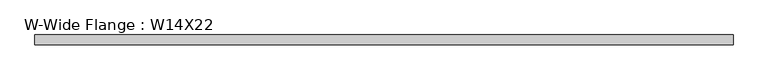
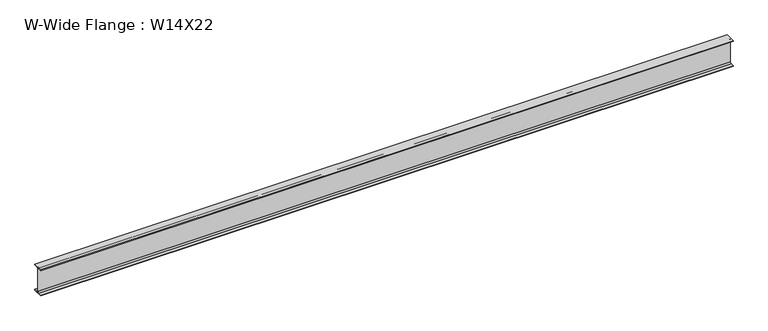
"""IFC4 building model written with IfcOpenShell, lengths in millimetres: beam geometry, W-Wide Flange : W14X22."""

import ifcopenshell
import ifcopenshell.guid

model = None  # the IFC model being written
_history = None  # IfcOwnerHistory: only IFC2X3 demands one
_inside = {}  # id of a spatial element -> (the spatial element, [elements in it])
_under = {}  # id of a project, library or spatial element -> (it, [spatial elements below it])
_declared = {}  # id of a project -> (the project, [libraries it declares])
_typed = {}  # id of a type object -> (the type object, [elements of that type])
_made_of = {}  # id of a material, layer set ... -> (it, [elements and type objects made of it])


def new_model(schema):
    """Start an empty IFC model of exactly this schema.

    Asked for "IFC4X3", IfcOpenShell would pick the latest addendum, in which some entities
    have other attributes; the version numbers below select the first issue.
    IFC2X3 requires an IfcOwnerHistory on every rooted entity: one is made here for all.
    """
    global model, _history
    if schema == "IFC4X3":
        model = ifcopenshell.file(schema_version=(4, 3, 0, 0))
    else:
        model = ifcopenshell.file(schema=schema)
    _inside.clear()
    _under.clear()
    _declared.clear()
    _typed.clear()
    _made_of.clear()
    _history = None
    if model.schema == "IFC2X3":
        org = make("IfcOrganization", Name="unknown")
        user = make(
            "IfcPersonAndOrganization",
            ThePerson=make("IfcPerson", FamilyName="unknown"),
            TheOrganization=org,
        )
        app = make(
            "IfcApplication",
            ApplicationDeveloper=org,
            Version="unknown",
            ApplicationFullName="unknown",
            ApplicationIdentifier="unknown",
        )
        _history = make(
            "IfcOwnerHistory",
            OwningUser=user,
            OwningApplication=app,
            ChangeAction="ADDED",
            CreationDate=0,
        )
    return model


def make(cls, **values):
    """One entity of the class cls with the attributes given. An attribute that is None is left unset."""
    return model.create_entity(
        cls, **{name: value for name, value in values.items() if value is not None}
    )


def rooted(cls, **values):
    """An entity with a GlobalId (a new one), such as an element, a storey or a relation."""
    return make(cls, GlobalId=ifcopenshell.guid.new(), OwnerHistory=_history, **values)


def si_unit(unit_type, name, prefix=None):
    """IfcSIUnit, for example si_unit("LENGTHUNIT", "METRE", prefix="MILLI")."""
    return make("IfcSIUnit", UnitType=unit_type, Prefix=prefix, Name=name)


def assignment(units):
    """IfcUnitAssignment: the units of a project."""
    return None if units is None else make("IfcUnitAssignment", Units=units)


def point(xyz):
    """IfcCartesianPoint."""
    return None if xyz is None else make("IfcCartesianPoint", Coordinates=xyz)


def direction(xyz):
    """IfcDirection."""
    return None if xyz is None else make("IfcDirection", DirectionRatios=xyz)


def frame(location, z_axis=None, x_axis=None):
    """IfcAxis2Placement3D, a coordinate frame: its origin and axes. An axis left out is left unset."""
    return make(
        "IfcAxis2Placement3D",
        Location=point(location),
        Axis=direction(z_axis),
        RefDirection=direction(x_axis),
    )


def frame_2d(location, x_axis=None):
    """IfcAxis2Placement2D, a coordinate frame in the plane: its origin and x axis."""
    return make(
        "IfcAxis2Placement2D", Location=point(location), RefDirection=direction(x_axis)
    )


def origin():
    """The frame at (0, 0, 0) with its axes left unset."""
    return frame((0.0, 0.0, 0.0))


def place(relative_to, where):
    """IfcLocalPlacement: puts the frame where relative to a parent placement (None: the world)."""
    return make(
        "IfcLocalPlacement", PlacementRelTo=relative_to, RelativePlacement=where
    )


def context(
    kind, dimensions, precision=None, world=None, true_north=None, identifier=None
):
    """IfcGeometricRepresentationContext, for example the 3D "Model" context."""
    return make(
        "IfcGeometricRepresentationContext",
        ContextIdentifier=identifier,
        ContextType=kind,
        CoordinateSpaceDimension=dimensions,
        Precision=precision,
        WorldCoordinateSystem=world,
        TrueNorth=true_north,
    )


def project(units=None, contexts=None):
    """IfcProject with its units and contexts."""
    return rooted(
        "IfcProject",
        Name="project",
        RepresentationContexts=contexts,
        UnitsInContext=assignment(units),
    )


def spatial(cls, under=None, at=None, **own):
    """A site, building, storey or space (cls), placed at a placement, below another one or the project."""
    s = rooted(cls, ObjectPlacement=at, **own)
    if under is not None:
        _under.setdefault(under.id(), (under, []))[1].append(s)
    return s


def polyline(points):
    """IfcPolyline through the points."""
    return make("IfcPolyline", Points=[point(p) for p in points])


def circle_curve(where, radius):
    """IfcCircle in the frame where."""
    return make("IfcCircle", Position=where, Radius=radius)


def trimmed(basis, trim1, trim2, sense, master):
    """IfcTrimmedCurve: the piece of a basis curve between two trims."""
    return make(
        "IfcTrimmedCurve",
        BasisCurve=basis,
        Trim1=trim1,
        Trim2=trim2,
        SenseAgreement=sense,
        MasterRepresentation=master,
    )


def segment(curve, same_sense, transition):
    """IfcCompositeCurveSegment."""
    return make(
        "IfcCompositeCurveSegment",
        Transition=transition,
        SameSense=same_sense,
        ParentCurve=curve,
    )


def composite_curve(segments, self_intersect=None):
    """IfcCompositeCurve: segments joined end to end."""
    return make("IfcCompositeCurve", Segments=segments, SelfIntersect=self_intersect)


def outline(outer, holes=None, kind="AREA"):
    """IfcArbitraryClosedProfileDef: a profile drawn as a closed curve; with holes, ...WithVoids."""
    if holes is None:
        return make("IfcArbitraryClosedProfileDef", ProfileType=kind, OuterCurve=outer)
    return make(
        "IfcArbitraryProfileDefWithVoids",
        ProfileType=kind,
        OuterCurve=outer,
        InnerCurves=holes,
    )


def extrude(swept, where, along, depth):
    """IfcExtrudedAreaSolid: the profile swept, set in the frame where, extruded along a direction by depth."""
    return make(
        "IfcExtrudedAreaSolid",
        SweptArea=swept,
        Position=where,
        ExtrudedDirection=direction(along),
        Depth=depth,
    )


def shape(context_of_items, identifier, shape_type, items):
    """IfcShapeRepresentation: the items that make up one representation, for example the "Body"."""
    return make(
        "IfcShapeRepresentation",
        ContextOfItems=context_of_items,
        RepresentationIdentifier=identifier,
        RepresentationType=shape_type,
        Items=items,
    )


def source(mapping_origin, context_of_items, identifier, shape_type, items):
    """IfcRepresentationMap: a shape defined once, which mapped items show again and again."""
    return make(
        "IfcRepresentationMap",
        MappingOrigin=mapping_origin,
        MappedRepresentation=shape(context_of_items, identifier, shape_type, items),
    )


def transform(
    local_origin,
    x_axis=None,
    y_axis=None,
    z_axis=None,
    scale=None,
    scale2=None,
    scale3=None,
    uniform=True,
):
    """IfcCartesianTransformationOperator3D, or its non-uniform kind. x_axis, y_axis, z_axis: its Axis1, 2, 3."""
    if uniform:
        return make(
            "IfcCartesianTransformationOperator3D",
            Axis1=direction(x_axis),
            Axis2=direction(y_axis),
            LocalOrigin=point(local_origin),
            Scale=scale,
            Axis3=direction(z_axis),
        )
    return make(
        "IfcCartesianTransformationOperator3DnonUniform",
        Axis1=direction(x_axis),
        Axis2=direction(y_axis),
        LocalOrigin=point(local_origin),
        Scale=scale,
        Axis3=direction(z_axis),
        Scale2=scale2,
        Scale3=scale3,
    )


def mapped(mapping_source, mapping_target):
    """IfcMappedItem: shows the shape of a source again, moved by a transform."""
    return make(
        "IfcMappedItem", MappingSource=mapping_source, MappingTarget=mapping_target
    )


def made_of(thing, what):
    """Note that an element or type object is made of a material, layer set ...; save() writes the relation."""
    if what is not None:
        _made_of.setdefault(what.id(), (what, []))[1].append(thing)
    return thing


def element(
    cls,
    number,
    at=None,
    inside=None,
    cuts=None,
    type_object=None,
    material=None,
    context=None,
    identifier="Body",
    shape_type=None,
    held_by="IfcProductDefinitionShape",
    body=None,
    shapes=None,
    **own,
):
    """One element of the class cls, such as IfcWall. Its Tag is "e" and its number.

    at: its placement. inside: the storey or other place that contains it. cuts: it is an
    opening in that element (IfcRelVoidsElement). A single representation is given by context,
    identifier, shape_type and body (its items); several are given by shapes. held_by: the class
    of the entity that holds the representations. save() writes the other relations.
    """
    e = rooted(cls, Tag="e%d" % number, ObjectPlacement=at, **own)
    if body is not None:
        shapes = [shape(context, identifier, shape_type, body)]
    if shapes is not None:
        e.Representation = make(held_by, Representations=shapes)
    if inside is not None:
        _inside.setdefault(inside.id(), (inside, []))[1].append(e)
    if cuts is not None:
        rooted(
            "IfcRelVoidsElement", RelatingBuildingElement=cuts, RelatedOpeningElement=e
        )
    if type_object is not None:
        _typed.setdefault(type_object.id(), (type_object, []))[1].append(e)
    return made_of(e, material)


def aggregate(whole, parts):
    """IfcRelAggregates: a whole, such as a stair, and the parts it consists of."""
    return rooted("IfcRelAggregates", RelatingObject=whole, RelatedObjects=parts)


def save(model, path):
    """Write the relations noted so far, then the file.

    IfcRelAggregates (storeys below a building ...), IfcRelContainedInSpatialStructure (elements
    in a storey), IfcRelDefinesByType, IfcRelAssociatesMaterial and IfcRelDeclares: one each for
    every whole, place, type object, material and project.
    """
    for whole, parts in _under.values():
        aggregate(whole, parts)
    for where, things in _inside.values():
        rooted(
            "IfcRelContainedInSpatialStructure",
            RelatedElements=things,
            RelatingStructure=where,
        )
    for kind, things in _typed.values():
        rooted("IfcRelDefinesByType", RelatedObjects=things, RelatingType=kind)
    for what, things in _made_of.values():
        rooted("IfcRelAssociatesMaterial", RelatedObjects=things, RelatingMaterial=what)
    for by, libraries in _declared.values():
        rooted("IfcRelDeclares", RelatingContext=by, RelatedDefinitions=libraries)
    model.write(path)


def w_wide_flange_w14x22_4ceff1ba(model_context):
    return source(origin(), model_context, "Body", "SweptSolid", [
        extrude(outline(composite_curve([segment(polyline([(63.5, -165.481), (63.5, -173.99), (-63.5, -173.99), (-63.5, -165.481), (-21.3995, -165.481)]), True, "CONTINUOUS"), segment(trimmed(circle_curve(frame_2d((-21.3995, -147.0025)), 18.4785), [point((-21.3995, -165.481))], [point((-2.921, -147.0025))], True, "CARTESIAN"), True, "CONTINUOUS"), segment(polyline([(-2.921, -147.0025), (-2.921, 147.0025)]), True, "CONTINUOUS"), segment(trimmed(circle_curve(frame_2d((-21.3995, 147.0025)), 18.4785), [point((-2.921, 147.0025))], [point((-21.3995, 165.481))], True, "CARTESIAN"), True, "CONTINUOUS"), segment(polyline([(-21.3995, 165.481), (-63.5, 165.481), (-63.5, 173.99), (63.5, 173.99), (63.5, 165.481), (21.3995, 165.481)]), True, "CONTINUOUS"), segment(trimmed(circle_curve(frame_2d((21.3995, 147.0025)), 18.4785), [point((21.3995, 165.481))], [point((2.921, 147.0025))], True, "CARTESIAN"), True, "CONTINUOUS"), segment(polyline([(2.921, 147.0025), (2.921, -147.0025)]), True, "CONTINUOUS"), segment(trimmed(circle_curve(frame_2d((21.3995, -147.0025)), 18.4785), [point((2.921, -147.0025))], [point((21.3995, -165.481))], True, "CARTESIAN"), True, "CONTINUOUS"), segment(polyline([(21.3995, -165.481), (63.5, -165.481)]), True, "CONTINUOUS")], self_intersect=False)), frame((-4381.4503906, 0.0, 0.0), z_axis=(1.0, 0.0, 0.0), x_axis=(0.0, 1.0, 0.0)), (0.0, 0.0, 1.0), 8826.1963906),
    ])


if __name__ == "__main__":
    model = new_model("IFC4")
    model_context = context("Model", 3, world=origin())
    ifc_project = project(units=[si_unit("LENGTHUNIT", "METRE", prefix="MILLI")], contexts=[model_context])
    site = spatial("IfcSite", under=ifc_project)
    building = spatial("IfcBuilding", under=site)
    placement = place(None, origin())
    w_wide_flange_w14x22_shape = w_wide_flange_w14x22_4ceff1ba(model_context)
    element("IfcBeam", 1, ObjectType="W-Wide Flange : W14X22", at=placement, inside=building, context=model_context, shape_type="MappedRepresentation", body=[
        mapped(w_wide_flange_w14x22_shape, transform((0.0, 0.0, 0.0), x_axis=(1.0, 0.0, 0.0), y_axis=(0.0, 1.0, 0.0), z_axis=(0.0, 0.0, 1.0))),
    ])
    save(model, "model.ifc")

# Revit data of these elements
# Type "W-Wide Flange : W14X22"
#   Assembly Code = "B10"
#   W = 22
#   Length [instance default] = 1524 mm
#   bf = 127 mm
#   d = 347.98 mm
#   k = 26.988 mm
#   k2 = 18.479 mm
#   tf = 8.509 mm
#   tw = 5.842 mm
#   A = 0.00418709 m²
#   Structural Material [instance default] = Steel ASTM A992
# Element 1 (IfcBeam, "W-Wide Flange : W14X22")
#   Structural Material = Aluminum, Anodized Red
#   Materials on its faces: "Aluminum, Anodized Red"
# Materials
#   "Steel ASTM A992": class "Metal", colour RGB 128 0 0, transparency 0, Description = "Structural steel 50ksi", Cost = 0
#   "Aluminum, Anodized Red": class "Metal", colour RGB 120 120 120, transparency 0, Description = "Anodized aluminum, red", Cost = 0
